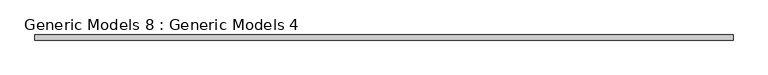
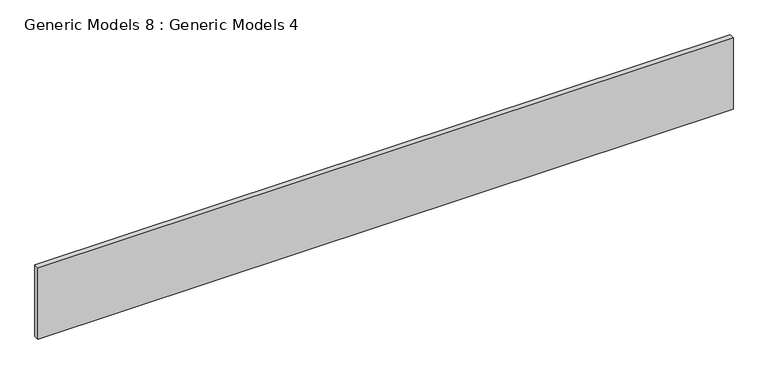
"""IFC4 building model written with IfcOpenShell, lengths in millimetres: proxy geometry, Generic Models 8 : Generic Models 4."""

from ifc_helpers import new_model, si_unit, frame, origin, place, context, project, spatial, polyline, outline, extrude, source, transform, mapped, element, save


def generic_models_8_generic_models_4_99fe06f1(model_context):
    return source(origin(), model_context, "Body", "SweptSolid", [
        extrude(outline(polyline([(24896.3074258, -8057.0818256), (24896.3074258, -8069.7818256), (23155.3573109, -8069.7818256), (23155.3573109, -8057.0818256), (24896.3074258, -8057.0818256)])), frame((0.0, 0.0, 123094.496), z_axis=(0.0, 0.0, 1.0), x_axis=(1.0, 0.0, 0.0)), (0.0, 0.0, 1.0), 189.1422763),
    ])


if __name__ == "__main__":
    model = new_model("IFC4")
    model_context = context("Model", 3, world=origin())
    ifc_project = project(units=[si_unit("LENGTHUNIT", "METRE", prefix="MILLI")], contexts=[model_context])
    site = spatial("IfcSite", under=ifc_project)
    building = spatial("IfcBuilding", under=site)
    placement = place(None, origin())
    generic_models_8_generic_models_4_shape = generic_models_8_generic_models_4_99fe06f1(model_context)
    element("IfcBuildingElementProxy", 1, Name="Generic Models 8 : Generic Models 4", ObjectType="Generic Models 8 : Generic Models 4", at=placement, inside=building, context=model_context, shape_type="MappedRepresentation", body=[
        mapped(generic_models_8_generic_models_4_shape, transform((0.0, 0.0, 0.0), x_axis=(1.0, 0.0, 0.0), y_axis=(0.0, 1.0, 0.0), z_axis=(0.0, 0.0, 1.0))),
    ])
    save(model, "model.ifc")

# Revit data of these elements
# Element 1 (IfcBuildingElementProxy, "Generic Models 8 : Generic Models 4")
#   Materials on its faces: "_CONCRETE EXPANSION JOINT - MINERAL FIBER"
# Materials
#   "_CONCRETE EXPANSION JOINT - MINERAL FIBER": class "Generic", colour RGB 190 220 196, transparency 0, Cost = 0
